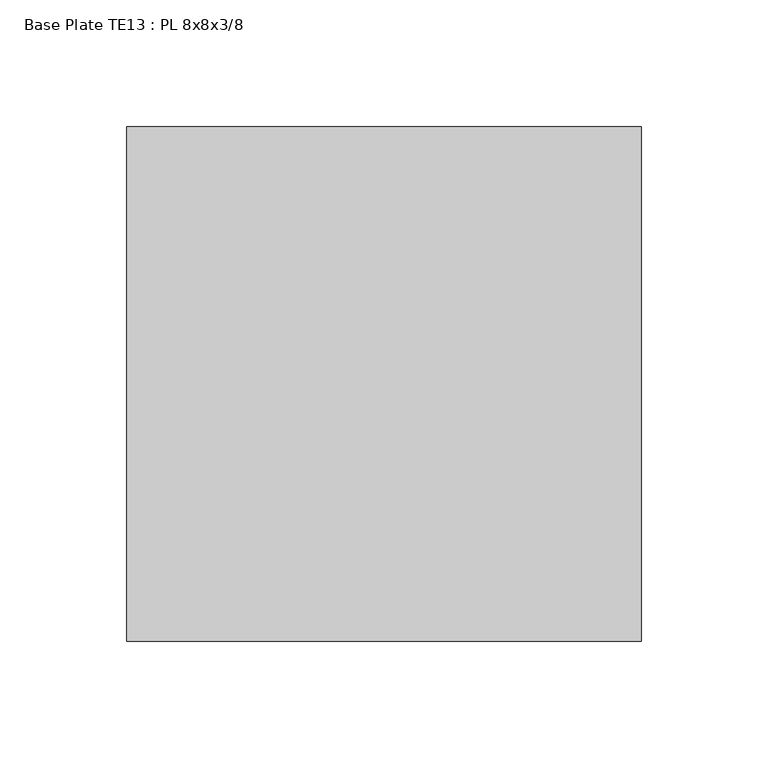
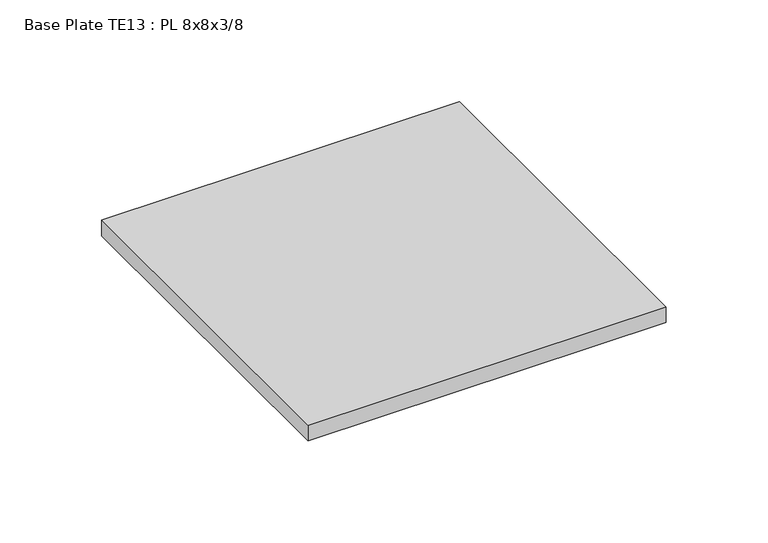
"""IFC4 building model written with IfcOpenShell, lengths in millimetres: proxy geometry, Base Plate TE13 : PL 8x8x3/8."""

from ifc_helpers import new_model, si_unit, frame, origin, place, context, project, spatial, polyline, outline, extrude, source, transform, mapped, element, save


def base_plate_te13_pl_8x8x3_8_c18328d5(model_context):
    return source(origin(), model_context, "Body", "SweptSolid", [
        extrude(outline(polyline([(590318.6599233, -536265.1913841), (590318.6599233, -536468.3913841), (590115.4599233, -536468.3913841), (590115.4599233, -536265.1913841), (590318.6599233, -536265.1913841)])), frame((0.0, 0.0, 19.05), z_axis=(0.0, 0.0, 1.0), x_axis=(1.0, 0.0, 0.0)), (0.0, 0.0, 1.0), 9.525),
    ])


if __name__ == "__main__":
    model = new_model("IFC4")
    model_context = context("Model", 3, world=origin())
    ifc_project = project(units=[si_unit("LENGTHUNIT", "METRE", prefix="MILLI")], contexts=[model_context])
    site = spatial("IfcSite", under=ifc_project)
    building = spatial("IfcBuilding", under=site)
    placement = place(None, origin())
    base_plate_te13_pl_8x8x3_8_shape = base_plate_te13_pl_8x8x3_8_c18328d5(model_context)
    element("IfcBuildingElementProxy", 1, Name="Base Plate TE13 : PL 8x8x3/8", ObjectType="Base Plate TE13 : PL 8x8x3/8", at=placement, inside=building, context=model_context, shape_type="MappedRepresentation", body=[
        mapped(base_plate_te13_pl_8x8x3_8_shape, transform((0.0, 0.0, 0.0), x_axis=(1.0, 0.0, 0.0), y_axis=(0.0, 1.0, 0.0), z_axis=(0.0, 0.0, 1.0))),
    ])
    save(model, "model.ifc")

# Revit data of these elements
# Element 1 (IfcBuildingElementProxy, "Base Plate TE13 : PL 8x8x3/8")
#   Materials on its faces: "GALV. STL BASE PLATE"
# Materials
#   "GALV. STL BASE PLATE": class "Generic", colour RGB 211 211 207, transparency 0, Cost = 0
